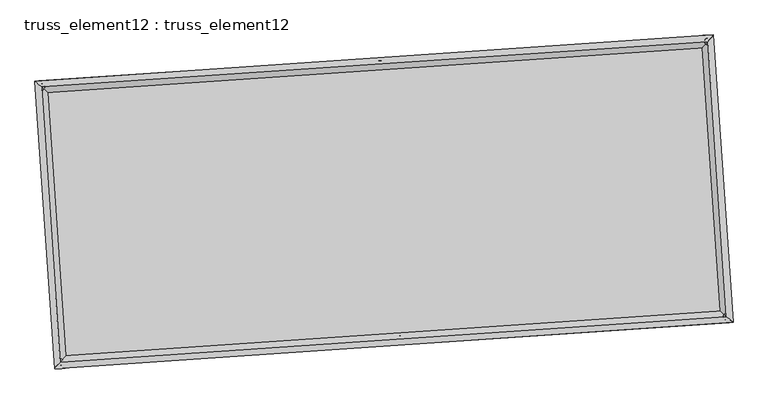
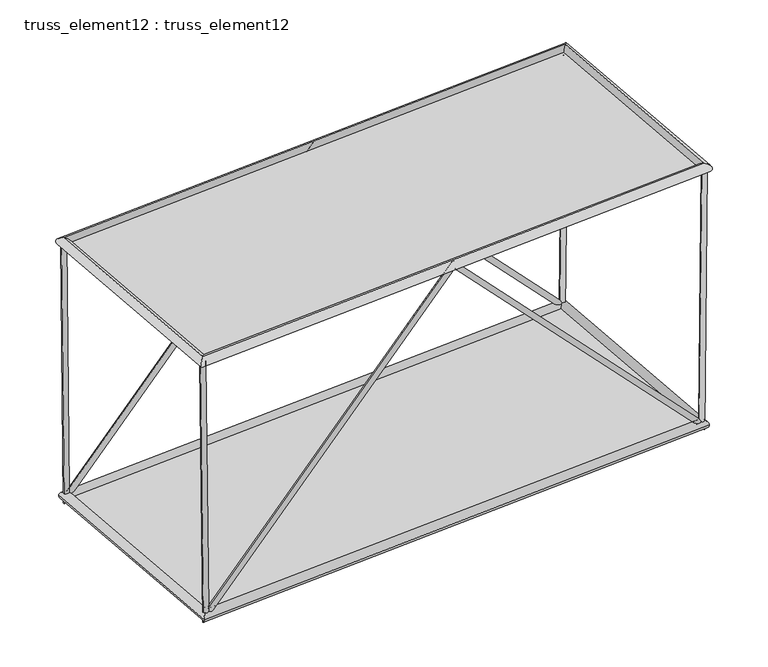
"""IFC4 building model written with IfcOpenShell, lengths in millimetres: plate geometry, truss_element12 : truss_element12."""

from ifc_helpers import new_model, si_unit, frame, origin, origin_with_axes, place, context, project, spatial, polyline, circle_curve, ellipse_curve, outline, extrude, source, transform, mapped, element, save
from ifc_brep_helpers import plane_surface, cylinder_surface, advanced_brep


def truss_element12_truss_element12_57bd624b(model_context):
    return source(origin(), model_context, "Body", "SolidModel", [
        advanced_brep(
        [(-3718.8834563, 2272.5458989, 5000.2471651), (-3817.9809982, 2259.1850197, 4999.1682339), (-3666.2639655, 2276.1338219, 122.8278962), (-3762.7229174, 2262.9528582, -122.8278962), (1063.2409993, 2598.6207869, 5071.8345956), (1063.6963469, 2592.0480409, 4927.5910062), (5793.6796472, 2921.1714162, 122.8345774), (5891.0813298, 2921.2090723, -122.8345774), (5845.3724971, 2924.6961552, 5000.2478695), (5945.3666498, 2924.9105819, 4999.187935)],
        [
            (0, 1, circle_curve(frame((-3768.4322273, 2265.8654593, 4999.7076995), z_axis=(-0.010787757166798292, -0.0007355761530998802, 0.9999415399027252), x_axis=(-0.1336089169721112, 0.9910338792341626, -0.0007124013101852261)), 50.0)),
            (1, 0, circle_curve(frame((-3768.4322273, 2265.8654593, 4999.7076995), z_axis=(-0.010787757166798292, -0.0007355761530998802, 0.9999415399027252), x_axis=(-0.1336089169721112, 0.9910338792341626, -0.0007124013101852261)), 50.0)),
            (0, 2),
            (2, 3, ellipse_curve(frame((-3714.4934414, 2269.54334, 0.0), z_axis=(-0.92779030394263, -0.06326249396471932, 0.36769961757854214), x_axis=(0.36684780320119337, 0.025013957181235023, 0.9299446172931988)), 132.3684791, 50.0)),
            (3, 1),
            (3, 2, ellipse_curve(frame((-3714.4934414, 2269.54334, 0.0), z_axis=(-0.92779030394263, -0.06326249396471932, 0.36769961757854214), x_axis=(0.36684780320119337, 0.025013957181235023, 0.9299446172931988)), 132.3684791, 50.0)),
            (2, 4),
            (4, 5, ellipse_curve(frame((1063.4686731, 2595.3344139, 4999.7128009), z_axis=(-0.9976833948456161, -0.06802823814488178, -4.9641008011428395e-05), x_axis=(4.952600945729314e-05, 3.3769903189971173e-06, -0.9999999987678851)), 72.2788404, 50.0)),
            (5, 3),
            (5, 4, ellipse_curve(frame((1063.4686731, 2595.3344139, 4999.7128009), z_axis=(-0.9976833948456161, -0.06802823814488178, -4.9641008011428395e-05), x_axis=(4.952600945729314e-05, 3.3769903189971173e-06, -0.9999999987678851)), 72.2788404, 50.0)),
            (4, 6),
            (6, 7, ellipse_curve(frame((5842.3804885, 2921.1902443, 0.0), z_axis=(-0.9277371610449604, -0.06325887035254266, -0.3678343041886623), x_axis=(-0.3669821777957838, -0.025023119674034488, 0.9298913509986222)), 132.383262, 50.0)),
            (7, 5),
            (7, 6, ellipse_curve(frame((5842.3804885, 2921.1902443, 0.0), z_axis=(-0.9277371610449604, -0.06325887035254266, -0.3678343041886623), x_axis=(-0.3669821777957838, -0.025023119674034488, 0.9298913509986222)), 132.383262, 50.0)),
            (8, 9, circle_curve(frame((5895.3695734, 2924.8033685, 4999.7179023), z_axis=(0.010597816986745603, 0.0007226248542524447, 0.9999435804526352), x_axis=(-0.002151805311608045, 0.9999974399630278, -0.0006998580510970341)), 50.0)),
            (9, 8, circle_curve(frame((5895.3695734, 2924.8033685, 4999.7179023), z_axis=(0.010597816986745603, 0.0007226248542524447, 0.9999435804526352), x_axis=(-0.002151805311608045, 0.9999974399630278, -0.0006998580510970341)), 50.0)),
            (6, 8),
            (9, 7),
        ],
        [
            plane_surface(frame((-3768.4322273, 2315.8654458, 4999.7444805), z_axis=(-0.010787757166800192, -0.0007355761530995395, 0.9999415399027252), x_axis=(0.9999418104546436, -7.935678691062265e-06, 0.010787754247981951))),
            cylinder_surface(frame((-3768.4322273, 2265.8654593, 4999.7076995), z_axis=(-0.010787757166798292, -0.0007355761530998802, 0.9999415399027252), x_axis=(-0.1336089169721112, 0.9910338792341626, -0.0007124013101852261)), 50.0),
            cylinder_surface(frame((-3714.4934414, 2269.54334, 0.0), z_axis=(-0.6901270755118669, -0.04705714186053672, -0.722156662397679), x_axis=(-0.020411387091029565, 0.9987523884926576, -0.04557457358255585)), 50.0),
            cylinder_surface(frame((1063.4686731, 2595.3344139, 4999.7128009), z_axis=(-0.690198603185899, -0.047062019060726955, 0.7220879825354816), x_axis=(-0.11534495483532443, 0.9922792293844502, -0.045579297123131184)), 50.0),
            plane_surface(frame((5895.3695734, 2874.8033816, 4999.7540355), z_axis=(0.010597816986746694, 0.0007226248542495468, 0.9999435804526353), x_axis=(0.9999438415606726, -7.6586760542341e-06, -0.010597814219416088))),
            cylinder_surface(frame((5842.3804885, 2921.1902443, 0.0), z_axis=(-0.010597816986745603, -0.0007226248542524447, -0.9999435804526352), x_axis=(-0.002151805311608045, 0.9999974399630278, -0.0006998580510970341)), 50.0),
        ],
        [
            (0, [[1, 2]]),
            (1, [[-1, 3, 4, 5]]),
            (1, [[-2, -5, 6, -3]]),
            (2, [[-4, 7, 8, 9]]),
            (2, [[-6, -9, 10, -7]]),
            (3, [[-8, 11, 12, 13]]),
            (3, [[-10, -13, 14, -11]]),
            (4, [[15, 16]]),
            (5, [[-12, 17, -16, 18]]),
            (5, [[-14, -18, -15, -17]]),
        ],
    ),
        advanced_brep(
        [(-3446.7705034, -1718.1876854, 5000.2471651), (-3545.8680453, -1731.5485646, 4999.1682339), (-3394.1510126, -1714.5997624, 122.8278962), (-3490.6099644, -1727.7807261, -122.8278962), (1335.3539522, -1392.1127974, 5071.8345956), (1335.8092998, -1398.6855434, 4927.5910062), (6065.7926001, -1069.5621681, 122.8345774), (6163.1942827, -1069.524512, -122.8345774), (6117.48545, -1066.0374291, 5000.2478695), (6217.4796027, -1065.8230024, 4999.187935)],
        [
            (0, 1, circle_curve(frame((-3496.3192743, -1724.868125, 4999.7076995), z_axis=(-0.010787757166798688, -0.0007355761530998968, 0.999941539902725), x_axis=(-0.13360891697211105, 0.9910338792341626, -0.0007124013101852608)), 50.0)),
            (1, 0, circle_curve(frame((-3496.3192743, -1724.868125, 4999.7076995), z_axis=(-0.010787757166798688, -0.0007355761530998968, 0.999941539902725), x_axis=(-0.13360891697211105, 0.9910338792341626, -0.0007124013101852608)), 50.0)),
            (0, 2),
            (2, 3, ellipse_curve(frame((-3442.3804885, -1721.1902443, 0.0), z_axis=(-0.9277903039426302, -0.0632624939647193, 0.36769961757854175), x_axis=(0.3668478032011929, 0.025013957181234996, 0.9299446172931988)), 132.3684791, 50.0)),
            (3, 1),
            (3, 2, ellipse_curve(frame((-3442.3804885, -1721.1902443, 0.0), z_axis=(-0.9277903039426302, -0.0632624939647193, 0.36769961757854175), x_axis=(0.3668478032011929, 0.025013957181234996, 0.9299446172931988)), 132.3684791, 50.0)),
            (2, 4),
            (4, 5, ellipse_curve(frame((1335.581626, -1395.3991704, 4999.7128009), z_axis=(-0.9976833948456163, -0.06802823814488179, -4.964100801174937e-05), x_axis=(4.952600945806187e-05, 3.37699031907399e-06, -0.9999999987678851)), 72.2788404, 50.0)),
            (5, 3),
            (5, 4, ellipse_curve(frame((1335.581626, -1395.3991704, 4999.7128009), z_axis=(-0.9976833948456163, -0.06802823814488179, -4.964100801174937e-05), x_axis=(4.952600945806187e-05, 3.37699031907399e-06, -0.9999999987678851)), 72.2788404, 50.0)),
            (4, 6),
            (6, 7, ellipse_curve(frame((6114.4934414, -1069.54334, 0.0), z_axis=(-0.9277371610449604, -0.06325887035254246, -0.36783430418866253), x_axis=(-0.366982177795784, -0.025023119674034606, 0.929891350998622)), 132.383262, 50.0)),
            (7, 5),
            (7, 6, ellipse_curve(frame((6114.4934414, -1069.54334, 0.0), z_axis=(-0.9277371610449604, -0.06325887035254246, -0.36783430418866253), x_axis=(-0.366982177795784, -0.025023119674034606, 0.929891350998622)), 132.383262, 50.0)),
            (8, 9, circle_curve(frame((6167.4825264, -1065.9302158, 4999.7179023), z_axis=(0.01059781698674539, 0.0007226248542522685, 0.9999435804526352), x_axis=(-0.00215180531160783, 0.9999974399630278, -0.0006998580510968606)), 50.0)),
            (9, 8, circle_curve(frame((6167.4825264, -1065.9302158, 4999.7179023), z_axis=(0.01059781698674539, 0.0007226248542522685, 0.9999435804526352), x_axis=(-0.00215180531160783, 0.9999974399630278, -0.0006998580510968606)), 50.0)),
            (6, 8),
            (9, 7),
        ],
        [
            plane_surface(frame((-3496.3192743, -1674.8681385, 4999.7444805), z_axis=(-0.010787757166800192, -0.0007355761530995395, 0.9999415399027252), x_axis=(0.9999418104546436, -7.935678691062265e-06, 0.010787754247981951))),
            cylinder_surface(frame((-3496.3192743, -1724.868125, 4999.7076995), z_axis=(-0.01078775716679869, -0.0007355761530998971, 0.9999415399027253), x_axis=(-0.13360891697211105, 0.9910338792341626, -0.0007124013101852608)), 50.0),
            cylinder_surface(frame((-3442.3804885, -1721.1902443, 0.0), z_axis=(-0.6901270755118669, -0.0470571418605367, -0.7221566623976791), x_axis=(-0.0204113870910296, 0.9987523884926577, -0.045574573582555795)), 50.0),
            cylinder_surface(frame((1335.581626, -1395.3991704, 4999.7128009), z_axis=(-0.6901986031858994, -0.047062019060727, 0.7220879825354812), x_axis=(-0.11534495483532436, 0.9922792293844502, -0.04557929712313114)), 50.0),
            plane_surface(frame((6167.4825264, -1115.9302027, 4999.7540355), z_axis=(0.010597816986746694, 0.0007226248542495459, 0.9999435804526353), x_axis=(0.9999438415606726, -7.658676054678189e-06, -0.010597814219416088))),
            cylinder_surface(frame((6114.4934414, -1069.54334, 0.0), z_axis=(-0.01059781698674539, -0.0007226248542522685, -0.9999435804526352), x_axis=(-0.00215180531160783, 0.9999974399630278, -0.0006998580510968606)), 50.0),
        ],
        [
            (0, [[1, 2]]),
            (1, [[-1, 3, 4, 5]]),
            (1, [[-2, -5, 6, -3]]),
            (2, [[-4, 7, 8, 9]]),
            (2, [[-6, -9, 10, -7]]),
            (3, [[-8, 11, 12, 13]]),
            (3, [[-10, -13, 14, -11]]),
            (4, [[15, 16]]),
            (5, [[-12, 17, -16, 18]]),
            (5, [[-14, -18, -15, -17]]),
        ],
    ),
        advanced_brep(
        [(-3496.3165918, -1724.8651518, 4909.7076996), (-3496.3219569, -1724.8710982, 5089.7076995), (-3768.4352886, 2265.8680408, 5089.7076995), (-3768.4291659, 2265.8628777, 4909.7076996), (5895.3720669, 2924.8063288, 5089.7179022), (5895.36708, 2924.8004082, 4909.7179023), (6167.4853985, -1065.9328102, 5089.7179022), (6167.4796542, -1065.9276213, 4909.7179023)],
        [
            (0, 1, ellipse_curve(frame((-3496.3192743, -1724.868125, 4999.7076995), z_axis=(-0.753571923405066, 0.6573654662781083, -7.448125030525588e-07), x_axis=(-0.6573654662776901, -0.7535719234054306, -7.448125030525935e-07)), 127.2792206, 90.0)),
            (1, 2),
            (2, 3, ellipse_curve(frame((-3768.4322273, 2265.8654593, 4999.7076995), z_axis=(-0.6573654662776901, -0.7535719234054307, -7.448125030526238e-07), x_axis=(0.7535719234050658, -0.6573654662781081, 7.448125030525892e-07)), 127.2792206, 90.0)),
            (3, 0),
            (1, 0, ellipse_curve(frame((-3496.3192743, -1724.868125, 4999.7076995), z_axis=(-0.753571923405066, 0.6573654662781083, -7.448125030525588e-07), x_axis=(-0.6573654662776901, -0.7535719234054306, -7.448125030525935e-07)), 127.2792206, 90.0)),
            (3, 2, ellipse_curve(frame((-3768.4322273, 2265.8654593, 4999.7076995), z_axis=(-0.6573654662776901, -0.7535719234054307, -7.448125030526238e-07), x_axis=(0.7535719234050658, -0.6573654662781081, 7.448125030525892e-07)), 127.2792206, 90.0)),
            (2, 4),
            (4, 5, ellipse_curve(frame((5895.3695734, 2924.8033685, 4999.7179023), z_axis=(-0.7535719234050661, 0.6573654662781081, -7.448125030526196e-07), x_axis=(-0.6573654662776902, -0.7535719234054307, -7.448125030525935e-07)), 127.2792206, 90.0)),
            (5, 3),
            (5, 4, ellipse_curve(frame((5895.3695734, 2924.8033685, 4999.7179023), z_axis=(-0.7535719234050661, 0.6573654662781081, -7.448125030526196e-07), x_axis=(-0.6573654662776902, -0.7535719234054307, -7.448125030525935e-07)), 127.2792206, 90.0)),
            (4, 6),
            (6, 7, ellipse_curve(frame((6167.4825264, -1065.9302158, 4999.7179023), z_axis=(0.6573654662776902, 0.7535719234054307, 7.44812503052563e-07), x_axis=(-0.7535719234050662, 0.6573654662781081, -7.448125030525893e-07)), 127.2792206, 90.0)),
            (7, 5),
            (7, 6, ellipse_curve(frame((6167.4825264, -1065.9302158, 4999.7179023), z_axis=(0.6573654662776902, 0.7535719234054307, 7.44812503052563e-07), x_axis=(-0.7535719234050662, 0.6573654662781081, -7.448125030525893e-07)), 127.2792206, 90.0)),
            (6, 1),
            (0, 7),
        ],
        [
            cylinder_surface(frame((-3496.3192743, -1724.868125, 4999.7076995), z_axis=(0.06802823822870147, -0.9976833960748767, 0.0), x_axis=(-0.9976833955645508, -0.06802823819390427, -3.198471076661545e-05)), 90.0),
            cylinder_surface(frame((-3768.4322273, 2265.8654593, 4999.7076995), z_axis=(-0.9976833960743233, -0.06802823822866153, -1.0533239432420484e-06), x_axis=(-0.06802823816365094, 0.9976833955998261, -3.093138682387732e-05)), 90.0),
            cylinder_surface(frame((5895.3695734, 2924.8033685, 4999.7179023), z_axis=(-0.06802823822870162, 0.9976833960748765, 0.0), x_axis=(0.9976833956295612, 0.06802823819833725, -2.9878062881139183e-05)), 90.0),
            cylinder_surface(frame((6167.4825264, -1065.9302158, 4999.7179023), z_axis=(0.9976833960743232, 0.0680282382286612, 1.0533239432420054e-06), x_axis=(0.0680282382286612, -0.9976833955953932, -3.093138682387733e-05)), 90.0),
        ],
        [
            (0, [[1, 2, 3, 4]]),
            (0, [[5, -4, 6, -2]]),
            (1, [[-3, 7, 8, 9]]),
            (1, [[-6, -9, 10, -7]]),
            (2, [[-8, 11, 12, 13]]),
            (2, [[-10, -13, 14, -11]]),
            (3, [[-12, 15, -1, 16]]),
            (3, [[-14, -16, -5, -15]]),
        ],
    ),
        advanced_brep(
        [(-3358.7115243, -1625.2761972, 0.0), (-3526.0494527, -1817.1042913, 0.0), (-3810.4074885, 2353.2123043, 0.0), (-3618.5793943, 2185.8743758, 0.0), (5926.0494527, 3017.1042913, 0.0), (5758.7115243, 2825.2761972, 0.0), (6210.4074885, -1153.2123043, 0.0), (6018.5793943, -985.8743758, 0.0)],
        [
            (0, 1, ellipse_curve(frame((-3442.3804885, -1721.1902443, 0.0), z_axis=(-0.7535719234054581, 0.6573654662780807, 0.0), x_axis=(-0.6573654662780808, -0.7535719234054581, 0.0)), 127.2792206, 90.0)),
            (1, 2),
            (2, 3, ellipse_curve(frame((-3714.4934414, 2269.54334, 0.0), z_axis=(-0.6573654662780807, -0.753571923405458, 0.0), x_axis=(0.7535719234054579, -0.6573654662780808, 0.0)), 127.2792206, 90.0)),
            (3, 0),
            (1, 0, ellipse_curve(frame((-3442.3804885, -1721.1902443, 0.0), z_axis=(-0.7535719234054581, 0.6573654662780807, 0.0), x_axis=(-0.6573654662780808, -0.7535719234054581, 0.0)), 127.2792206, 90.0)),
            (3, 2, ellipse_curve(frame((-3714.4934414, 2269.54334, 0.0), z_axis=(-0.6573654662780807, -0.753571923405458, 0.0), x_axis=(0.7535719234054579, -0.6573654662780808, 0.0)), 127.2792206, 90.0)),
            (2, 4),
            (4, 5, ellipse_curve(frame((5842.3804885, 2921.1902443, 0.0), z_axis=(-0.7535719234054582, 0.6573654662780806, 0.0), x_axis=(-0.6573654662780805, -0.7535719234054583, 0.0)), 127.2792206, 90.0)),
            (5, 3),
            (5, 4, ellipse_curve(frame((5842.3804885, 2921.1902443, 0.0), z_axis=(-0.7535719234054582, 0.6573654662780806, 0.0), x_axis=(-0.6573654662780805, -0.7535719234054583, 0.0)), 127.2792206, 90.0)),
            (4, 6),
            (6, 7, ellipse_curve(frame((6114.4934414, -1069.54334, 0.0), z_axis=(0.6573654662780806, 0.7535719234054581, 0.0), x_axis=(-0.7535719234054581, 0.6573654662780806, 0.0)), 127.2792206, 90.0)),
            (7, 5),
            (7, 6, ellipse_curve(frame((6114.4934414, -1069.54334, 0.0), z_axis=(0.6573654662780806, 0.7535719234054581, 0.0), x_axis=(-0.7535719234054581, 0.6573654662780806, 0.0)), 127.2792206, 90.0)),
            (6, 1),
            (0, 7),
        ],
        [
            cylinder_surface(frame((-3442.3804885, -1721.1902443, 0.0), z_axis=(0.06802823822870274, -0.9976833960748764, 0.0), x_axis=(-0.9976833960748764, -0.06802823822870274, 0.0)), 90.0),
            cylinder_surface(frame((-3714.4934414, 2269.54334, 0.0), z_axis=(-0.9976833960748767, -0.06802823822870008, 0.0), x_axis=(-0.06802823822870008, 0.9976833960748767, 0.0)), 90.0),
            cylinder_surface(frame((5842.3804885, 2921.1902443, 0.0), z_axis=(-0.06802823822870283, 0.9976833960748764, 0.0), x_axis=(0.9976833960748764, 0.06802823822870283, 0.0)), 90.0),
            cylinder_surface(frame((6114.4934414, -1069.54334, 0.0), z_axis=(0.9976833960748767, 0.06802823822870016, 0.0), x_axis=(0.06802823822870016, -0.9976833960748767, 0.0)), 90.0),
        ],
        [
            (0, [[1, 2, 3, 4]]),
            (0, [[5, -4, 6, -2]]),
            (1, [[-3, 7, 8, 9]]),
            (1, [[-6, -9, 10, -7]]),
            (2, [[-8, 11, 12, 13]]),
            (2, [[-10, -13, 14, -11]]),
            (3, [[-12, 15, -1, 16]]),
            (3, [[-14, -16, -5, -15]]),
        ],
    ),
        extrude(outline(polyline([(-3442.3804885, -1721.1902443), (-3714.4934414, 2269.54334), (5842.3804885, 2921.1902443), (6114.4934414, -1069.54334), (-3442.3804885, -1721.1902443)])), origin_with_axes(), (0.0, 0.0, 1.0), 20.0),
        extrude(outline(polyline([(-2000.0, 4843.1204922), (2000.0, 4843.1204923), (1999.9999999, -4843.1204923), (-2000.0000001, -4843.1204924), (-2000.0, 4843.1204922)])), frame((1199.5251495, 599.9676218, 4999.7128009), z_axis=(-1.0508838088606855e-06, -7.165577214286503e-08, 0.9999999999994453), x_axis=(-0.06802823822870262, 0.9976833960748765, 0.0)), (0.0, 0.0, 1.0), 20.0),
    ])


if __name__ == "__main__":
    model = new_model("IFC4")
    model_context = context("Model", 3, world=origin())
    ifc_project = project(units=[si_unit("LENGTHUNIT", "METRE", prefix="MILLI")], contexts=[model_context])
    site = spatial("IfcSite", under=ifc_project)
    building = spatial("IfcBuilding", under=site)
    placement = place(None, origin())
    truss_element12_truss_element12_shape = truss_element12_truss_element12_57bd624b(model_context)
    element("IfcPlate", 1, ObjectType="truss_element12 : truss_element12", at=placement, inside=building, context=model_context, shape_type="MappedRepresentation", body=[
        mapped(truss_element12_truss_element12_shape, transform((0.0, 0.0, 0.0), x_axis=(1.0, 0.0, 0.0), y_axis=(0.0, 1.0, 0.0), z_axis=(0.0, 0.0, 1.0))),
    ])
    save(model, "model.ifc")

# Revit data of these elements
# Type "truss_element12 : truss_element12"
#   steellbar1 = 90 mm
#   steelbar2 = 50 mm
#   offset1 = 5000 mm
#   M = Default Roof
# Element 1 (IfcPlate, "truss_element12 : truss_element12")
#   Materials on its faces: "Default Roof"
# Materials
#   "Default Roof": class "Miscellaneous", colour RGB 0 127 0, transparency 0, Comments = "Rendering appearance not upgraded Rendering appearance not upgraded ", Cost = 0
